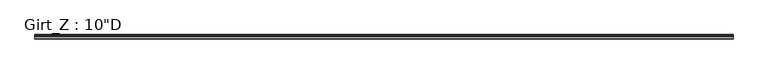
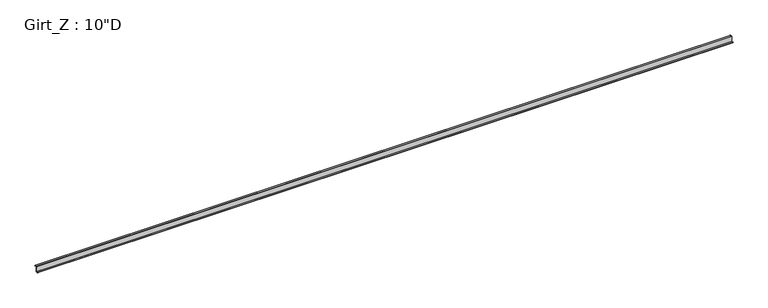
"""IFC4 building model written with IfcOpenShell, lengths in millimetres: beam geometry."""

from ifc_helpers import new_model, si_unit, point, frame, frame_2d, origin, place, context, project, spatial, polyline, circle_curve, trimmed, segment, composite_curve, outline, extrude, source, transform, mapped, element, save


def beam_638428f9(model_context):
    return source(origin(), model_context, "Body", "SweptSolid", [
        extrude(outline(composite_curve([segment(polyline([(77.9859375, 127.0), (90.2310415, 112.4068534), (88.1028742, 110.621109), (76.6904765, 124.221875), (3.3005807, 124.221875)]), True, "CONTINUOUS"), segment(trimmed(circle_curve(frame_2d((3.3741066, 122.2381931)), 1.9850441), [point((3.3005807, 124.221875))], [point((1.3890625, 122.2381931))], True, "CARTESIAN"), True, "CONTINUOUS"), segment(polyline([(1.3890625, 122.2381931), (1.3890625, -127.0), (-84.3359375, -127.0), (-96.5810415, -112.4068534), (-94.4528742, -110.621109), (-83.0404765, -124.221875), (-3.2694106, -124.221875)]), True, "CONTINUOUS"), segment(trimmed(circle_curve(frame_2d((-3.3748024, -122.2389339)), 1.9857399), [point((-3.2694106, -124.221875))], [point((-1.3890625, -122.2389339))], True, "CARTESIAN"), True, "CONTINUOUS"), segment(polyline([(-1.3890625, -122.2389339), (-1.3890625, 122.2375)]), True, "CONTINUOUS"), segment(trimmed(circle_curve(frame_2d((3.3734375, 122.2375)), 4.7625), [point((-1.3890625, 122.2375))], [point((3.3734375, 127.0))], False, "CARTESIAN"), True, "CONTINUOUS"), segment(polyline([(3.3734375, 127.0), (77.9859375, 127.0)]), True, "CONTINUOUS")], self_intersect=False)), frame((-15640.05, 0.0, 0.0), z_axis=(1.0, 0.0, 0.0), x_axis=(0.0, 1.0, 0.0)), (0.0, 0.0, 1.0), 31121.35),
    ])


if __name__ == "__main__":
    model = new_model("IFC4")
    model_context = context("Model", 3, world=origin())
    ifc_project = project(units=[si_unit("LENGTHUNIT", "METRE", prefix="MILLI")], contexts=[model_context])
    site = spatial("IfcSite", under=ifc_project)
    building = spatial("IfcBuilding", under=site)
    placement = place(None, origin())
    beam_shape = beam_638428f9(model_context)
    element("IfcBeam", 1, ObjectType="Girt_Z : 10\"D", at=placement, inside=building, context=model_context, shape_type="MappedRepresentation", body=[
        mapped(beam_shape, transform((0.0, 0.0, 0.0), x_axis=(1.0, 0.0, 0.0), y_axis=(0.0, 1.0, 0.0), z_axis=(0.0, 0.0, 1.0))),
    ])
    save(model, "model.ifc")

# Revit data of these elements
# Type "Girt_Z : 10\"D"
#   half leg = 0' - 1 11/16"
#   Web_Thickness = 0' - 0 7/64"
#   Length [instance default] = 10' - 0"
#   Leg_2 = 0' - 3 3/8"
#   Leg_1 = 0' - 3 1/8"
#   Height = 0' - 10"
#   Structural Material [instance default] = none
# Element 1 (IfcBeam, "Girt_Z : 10\"D")
#   Structural Material = STRUCTURAL STEEL - SEE STRUCT. DWGS
#   Materials on its faces: "STRUCTURAL STEEL - SEE STRUCT. DWGS"
# Materials
#   "STRUCTURAL STEEL - SEE STRUCT. DWGS": class "Metal", colour RGB 137 146 153, transparency 0, Description = "Steel, mill finish", Cost = 0
